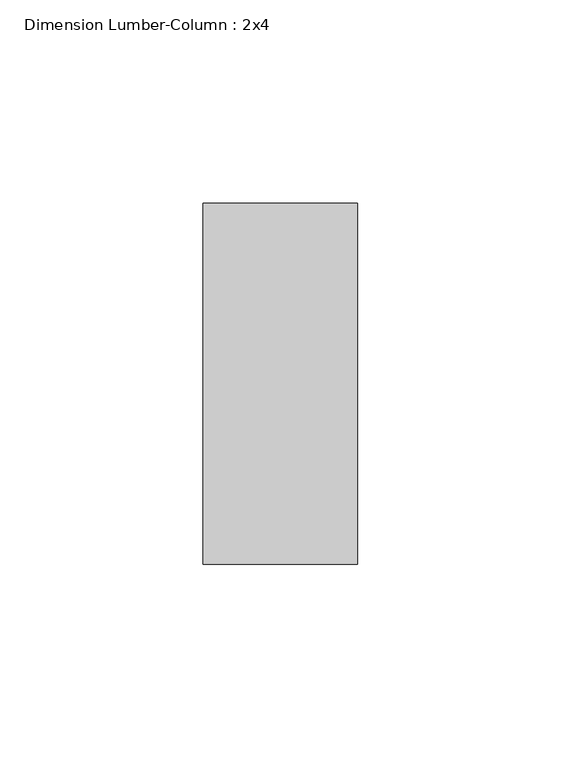
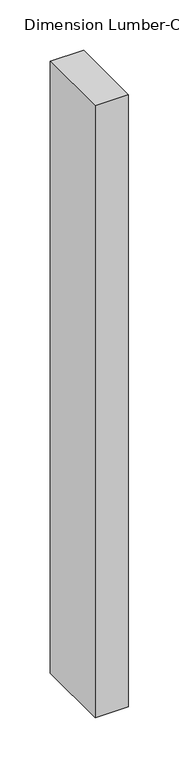
"""IFC4 building model written with IfcOpenShell, lengths in millimetres: column geometry, Dimension Lumber-Column : 2x4."""

from ifc_helpers import new_model, si_unit, frame, origin, place, context, project, spatial, polyline, outline, extrude, source, transform, mapped, element, save


def dimension_lumber_column_2x4_35883525(model_context):
    return source(origin(), model_context, "Body", "SweptSolid", [
        extrude(outline(polyline([(19.05, 44.45), (19.05, -44.45), (-19.05, -44.45), (-19.05, 44.45), (19.05, 44.45)])), frame((0.0, 0.0, 56.35625), z_axis=(0.0, 0.0, 1.0), x_axis=(1.0, 0.0, 0.0)), (0.0, 0.0, 1.0), 742.553125),
    ])


if __name__ == "__main__":
    model = new_model("IFC4")
    model_context = context("Model", 3, world=origin())
    ifc_project = project(units=[si_unit("LENGTHUNIT", "METRE", prefix="MILLI")], contexts=[model_context])
    site = spatial("IfcSite", under=ifc_project)
    building = spatial("IfcBuilding", under=site)
    placement = place(None, origin())
    dimension_lumber_column_2x4_shape = dimension_lumber_column_2x4_35883525(model_context)
    element("IfcColumn", 1, ObjectType="Dimension Lumber-Column : 2x4", at=placement, inside=building, context=model_context, shape_type="MappedRepresentation", body=[
        mapped(dimension_lumber_column_2x4_shape, transform((0.0, 0.0, 0.0), x_axis=(1.0, 0.0, 0.0), y_axis=(0.0, 1.0, 0.0), z_axis=(0.0, 0.0, 1.0))),
    ])
    save(model, "model.ifc")

# Revit data of these elements
# Type "Dimension Lumber-Column : 2x4"
#   Int Type = "Interior"
#   Assembly Code = "B10"
#   Cost = 8.05
#   A = 0.0364583 SF
#   b = 0' - 1 1/2"
#   d = 0' - 3 1/2"
#   Structural Material [instance default] = Softwood, Lumber
# Element 1 (IfcColumn, "Dimension Lumber-Column : 2x4")
#   Structural Material = Douglas Fir #2
#   Materials on its faces: "Douglas Fir #2"
# Materials
#   "Softwood, Lumber": class "Wood", colour RGB 223 192 134, transparency 0, Description = "Pinus Echinata", Cost = 0
#   "Douglas Fir #2": class "Wood", colour RGB 223 192 134, transparency 0, Description = "Pinus Echinata", Cost = 0
